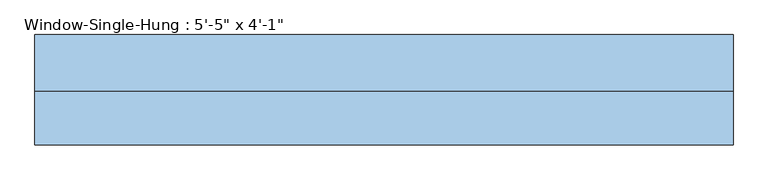
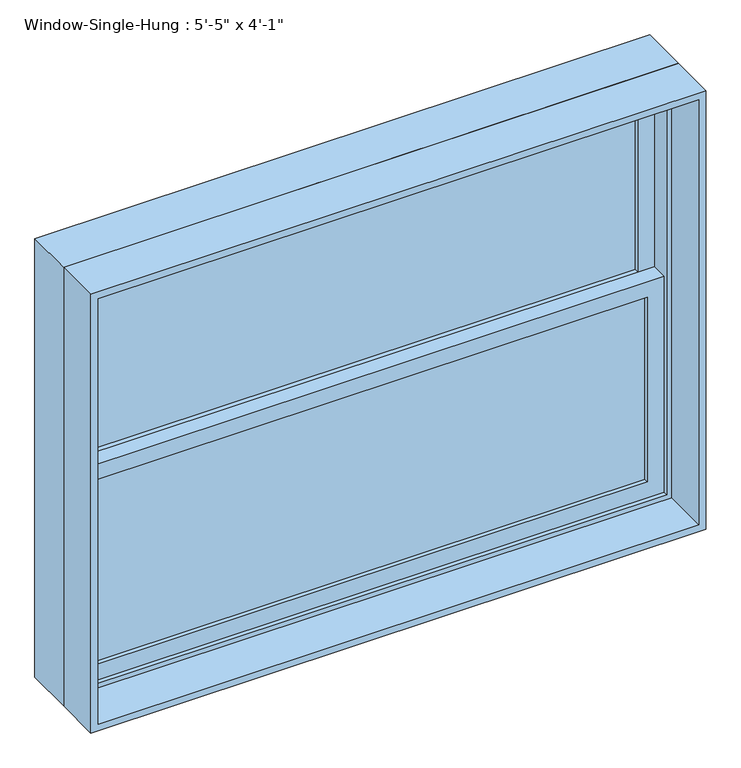
"""IFC4 building model written with IfcOpenShell, lengths in millimetres: window geometry."""

import ifcopenshell
import ifcopenshell.guid

model = None  # the IFC model being written
_history = None  # IfcOwnerHistory: only IFC2X3 demands one
_inside = {}  # id of a spatial element -> (the spatial element, [elements in it])
_under = {}  # id of a project, library or spatial element -> (it, [spatial elements below it])
_declared = {}  # id of a project -> (the project, [libraries it declares])
_typed = {}  # id of a type object -> (the type object, [elements of that type])
_made_of = {}  # id of a material, layer set ... -> (it, [elements and type objects made of it])


def new_model(schema):
    """Start an empty IFC model of exactly this schema.

    Asked for "IFC4X3", IfcOpenShell would pick the latest addendum, in which some entities
    have other attributes; the version numbers below select the first issue.
    IFC2X3 requires an IfcOwnerHistory on every rooted entity: one is made here for all.
    """
    global model, _history
    if schema == "IFC4X3":
        model = ifcopenshell.file(schema_version=(4, 3, 0, 0))
    else:
        model = ifcopenshell.file(schema=schema)
    _inside.clear()
    _under.clear()
    _declared.clear()
    _typed.clear()
    _made_of.clear()
    _history = None
    if model.schema == "IFC2X3":
        org = make("IfcOrganization", Name="unknown")
        user = make(
            "IfcPersonAndOrganization",
            ThePerson=make("IfcPerson", FamilyName="unknown"),
            TheOrganization=org,
        )
        app = make(
            "IfcApplication",
            ApplicationDeveloper=org,
            Version="unknown",
            ApplicationFullName="unknown",
            ApplicationIdentifier="unknown",
        )
        _history = make(
            "IfcOwnerHistory",
            OwningUser=user,
            OwningApplication=app,
            ChangeAction="ADDED",
            CreationDate=0,
        )
    return model


def make(cls, **values):
    """One entity of the class cls with the attributes given. An attribute that is None is left unset."""
    return model.create_entity(
        cls, **{name: value for name, value in values.items() if value is not None}
    )


def rooted(cls, **values):
    """An entity with a GlobalId (a new one), such as an element, a storey or a relation."""
    return make(cls, GlobalId=ifcopenshell.guid.new(), OwnerHistory=_history, **values)


def si_unit(unit_type, name, prefix=None):
    """IfcSIUnit, for example si_unit("LENGTHUNIT", "METRE", prefix="MILLI")."""
    return make("IfcSIUnit", UnitType=unit_type, Prefix=prefix, Name=name)


def assignment(units):
    """IfcUnitAssignment: the units of a project."""
    return None if units is None else make("IfcUnitAssignment", Units=units)


def point(xyz):
    """IfcCartesianPoint."""
    return None if xyz is None else make("IfcCartesianPoint", Coordinates=xyz)


def direction(xyz):
    """IfcDirection."""
    return None if xyz is None else make("IfcDirection", DirectionRatios=xyz)


def frame(location, z_axis=None, x_axis=None):
    """IfcAxis2Placement3D, a coordinate frame: its origin and axes. An axis left out is left unset."""
    return make(
        "IfcAxis2Placement3D",
        Location=point(location),
        Axis=direction(z_axis),
        RefDirection=direction(x_axis),
    )


def origin():
    """The frame at (0, 0, 0) with its axes left unset."""
    return frame((0.0, 0.0, 0.0))


def place(relative_to, where):
    """IfcLocalPlacement: puts the frame where relative to a parent placement (None: the world)."""
    return make(
        "IfcLocalPlacement", PlacementRelTo=relative_to, RelativePlacement=where
    )


def context(
    kind, dimensions, precision=None, world=None, true_north=None, identifier=None
):
    """IfcGeometricRepresentationContext, for example the 3D "Model" context."""
    return make(
        "IfcGeometricRepresentationContext",
        ContextIdentifier=identifier,
        ContextType=kind,
        CoordinateSpaceDimension=dimensions,
        Precision=precision,
        WorldCoordinateSystem=world,
        TrueNorth=true_north,
    )


def project(units=None, contexts=None):
    """IfcProject with its units and contexts."""
    return rooted(
        "IfcProject",
        Name="project",
        RepresentationContexts=contexts,
        UnitsInContext=assignment(units),
    )


def spatial(cls, under=None, at=None, **own):
    """A site, building, storey or space (cls), placed at a placement, below another one or the project."""
    s = rooted(cls, ObjectPlacement=at, **own)
    if under is not None:
        _under.setdefault(under.id(), (under, []))[1].append(s)
    return s


def polyline(points):
    """IfcPolyline through the points."""
    return make("IfcPolyline", Points=[point(p) for p in points])


def outline(outer, holes=None, kind="AREA"):
    """IfcArbitraryClosedProfileDef: a profile drawn as a closed curve; with holes, ...WithVoids."""
    if holes is None:
        return make("IfcArbitraryClosedProfileDef", ProfileType=kind, OuterCurve=outer)
    return make(
        "IfcArbitraryProfileDefWithVoids",
        ProfileType=kind,
        OuterCurve=outer,
        InnerCurves=holes,
    )


def extrude(swept, where, along, depth):
    """IfcExtrudedAreaSolid: the profile swept, set in the frame where, extruded along a direction by depth."""
    return make(
        "IfcExtrudedAreaSolid",
        SweptArea=swept,
        Position=where,
        ExtrudedDirection=direction(along),
        Depth=depth,
    )


def shape(context_of_items, identifier, shape_type, items):
    """IfcShapeRepresentation: the items that make up one representation, for example the "Body"."""
    return make(
        "IfcShapeRepresentation",
        ContextOfItems=context_of_items,
        RepresentationIdentifier=identifier,
        RepresentationType=shape_type,
        Items=items,
    )


def source(mapping_origin, context_of_items, identifier, shape_type, items):
    """IfcRepresentationMap: a shape defined once, which mapped items show again and again."""
    return make(
        "IfcRepresentationMap",
        MappingOrigin=mapping_origin,
        MappedRepresentation=shape(context_of_items, identifier, shape_type, items),
    )


def transform(
    local_origin,
    x_axis=None,
    y_axis=None,
    z_axis=None,
    scale=None,
    scale2=None,
    scale3=None,
    uniform=True,
):
    """IfcCartesianTransformationOperator3D, or its non-uniform kind. x_axis, y_axis, z_axis: its Axis1, 2, 3."""
    if uniform:
        return make(
            "IfcCartesianTransformationOperator3D",
            Axis1=direction(x_axis),
            Axis2=direction(y_axis),
            LocalOrigin=point(local_origin),
            Scale=scale,
            Axis3=direction(z_axis),
        )
    return make(
        "IfcCartesianTransformationOperator3DnonUniform",
        Axis1=direction(x_axis),
        Axis2=direction(y_axis),
        LocalOrigin=point(local_origin),
        Scale=scale,
        Axis3=direction(z_axis),
        Scale2=scale2,
        Scale3=scale3,
    )


def mapped(mapping_source, mapping_target):
    """IfcMappedItem: shows the shape of a source again, moved by a transform."""
    return make(
        "IfcMappedItem", MappingSource=mapping_source, MappingTarget=mapping_target
    )


def made_of(thing, what):
    """Note that an element or type object is made of a material, layer set ...; save() writes the relation."""
    if what is not None:
        _made_of.setdefault(what.id(), (what, []))[1].append(thing)
    return thing


def element(
    cls,
    number,
    at=None,
    inside=None,
    cuts=None,
    type_object=None,
    material=None,
    context=None,
    identifier="Body",
    shape_type=None,
    held_by="IfcProductDefinitionShape",
    body=None,
    shapes=None,
    **own,
):
    """One element of the class cls, such as IfcWall. Its Tag is "e" and its number.

    at: its placement. inside: the storey or other place that contains it. cuts: it is an
    opening in that element (IfcRelVoidsElement). A single representation is given by context,
    identifier, shape_type and body (its items); several are given by shapes. held_by: the class
    of the entity that holds the representations. save() writes the other relations.
    """
    e = rooted(cls, Tag="e%d" % number, ObjectPlacement=at, **own)
    if body is not None:
        shapes = [shape(context, identifier, shape_type, body)]
    if shapes is not None:
        e.Representation = make(held_by, Representations=shapes)
    if inside is not None:
        _inside.setdefault(inside.id(), (inside, []))[1].append(e)
    if cuts is not None:
        rooted(
            "IfcRelVoidsElement", RelatingBuildingElement=cuts, RelatedOpeningElement=e
        )
    if type_object is not None:
        _typed.setdefault(type_object.id(), (type_object, []))[1].append(e)
    return made_of(e, material)


def aggregate(whole, parts):
    """IfcRelAggregates: a whole, such as a stair, and the parts it consists of."""
    return rooted("IfcRelAggregates", RelatingObject=whole, RelatedObjects=parts)


def save(model, path):
    """Write the relations noted so far, then the file.

    IfcRelAggregates (storeys below a building ...), IfcRelContainedInSpatialStructure (elements
    in a storey), IfcRelDefinesByType, IfcRelAssociatesMaterial and IfcRelDeclares: one each for
    every whole, place, type object, material and project.
    """
    for whole, parts in _under.values():
        aggregate(whole, parts)
    for where, things in _inside.values():
        rooted(
            "IfcRelContainedInSpatialStructure",
            RelatedElements=things,
            RelatingStructure=where,
        )
    for kind, things in _typed.values():
        rooted("IfcRelDefinesByType", RelatedObjects=things, RelatingType=kind)
    for what, things in _made_of.values():
        rooted("IfcRelAssociatesMaterial", RelatedObjects=things, RelatingMaterial=what)
    for by, libraries in _declared.values():
        rooted("IfcRelDeclares", RelatingContext=by, RelatedDefinitions=libraries)
    model.write(path)


def window_21bbe75a(model_context):
    return source(origin(), model_context, "Body", "SweptSolid", [
        extrude(outline(polyline([(749.3, 50.8), (749.3, 44.45), (-749.3, 44.45), (-749.3, 50.8), (749.3, 50.8)])), frame((0.0, 0.0, 990.6), z_axis=(0.0, 0.0, 1.0), x_axis=(1.0, 0.0, 0.0)), (0.0, 0.0, 1.0), 523.875),
        extrude(outline(polyline([(-749.3, 38.1), (749.3, 38.1), (749.3, 31.75), (-749.3, 31.75), (-749.3, 38.1)])), frame((0.0, 0.0, 990.6), z_axis=(0.0, 0.0, 1.0), x_axis=(1.0, 0.0, 0.0)), (0.0, 0.0, 1.0), 523.875),
        extrude(outline(polyline([(749.3, 95.25), (749.3, 88.9), (-749.3, 88.9), (-749.3, 95.25), (749.3, 95.25)])), frame((0.0, 0.0, 1558.925), z_axis=(0.0, 0.0, 1.0), x_axis=(1.0, 0.0, 0.0)), (0.0, 0.0, 1.0), 523.875),
        extrude(outline(polyline([(-749.3, 82.55), (749.3, 82.55), (749.3, 76.2), (-749.3, 76.2), (-749.3, 82.55)])), frame((0.0, 0.0, 1558.925), z_axis=(0.0, 0.0, 1.0), x_axis=(1.0, 0.0, 0.0)), (0.0, 0.0, 1.0), 523.875),
        extrude(outline(polyline([(1558.925, -793.75), (946.15, -793.75), (946.15, 793.75), (1558.925, 793.75), (1558.925, -793.75)]), holes=[polyline([(1514.475, 749.3), (990.6, 749.3), (990.6, -749.3), (1514.475, -749.3), (1514.475, 749.3)])]), frame((0.0, 19.05, 0.0), z_axis=(0.0, 1.0, 0.0), x_axis=(0.0, 0.0, 1.0)), (0.0, 0.0, 1.0), 44.45),
        extrude(outline(polyline([(2127.25, -793.75), (1514.475, -793.75), (1514.475, 793.75), (2127.25, 793.75), (2127.25, -793.75)]), holes=[polyline([(2082.8, 749.3), (1558.925, 749.3), (1558.925, -749.3), (2082.8, -749.3), (2082.8, 749.3)])]), frame((0.0, 63.5, 0.0), z_axis=(0.0, 1.0, 0.0), x_axis=(0.0, 0.0, 1.0)), (0.0, 0.0, 1.0), 44.45),
        extrude(outline(polyline([(2159.0, -825.5), (914.4, -825.5), (914.4, 825.5), (2159.0, 825.5), (2159.0, -825.5)]), holes=[polyline([(2127.25, 793.75), (946.15, 793.75), (946.15, -793.75), (2127.25, -793.75), (2127.25, 793.75)])]), frame((0.0, 6.35, 0.0), z_axis=(0.0, 1.0, 0.0), x_axis=(0.0, 0.0, 1.0)), (0.0, 0.0, 1.0), 133.35),
        extrude(outline(polyline([(2159.0, 825.5), (2159.0, -825.5), (914.4, -825.5), (914.4, 825.5), (2159.0, 825.5)]), holes=[polyline([(2139.95, 806.45), (933.45, 806.45), (933.45, -806.45), (2139.95, -806.45), (2139.95, 806.45)])]), frame((0.0, -120.65, 0.0), z_axis=(0.0, 1.0, 0.0), x_axis=(0.0, 0.0, 1.0)), (0.0, 0.0, 1.0), 127.0),
    ])


if __name__ == "__main__":
    model = new_model("IFC4")
    model_context = context("Model", 3, world=origin())
    ifc_project = project(units=[si_unit("LENGTHUNIT", "METRE", prefix="MILLI")], contexts=[model_context])
    site = spatial("IfcSite", under=ifc_project)
    building = spatial("IfcBuilding", under=site)
    placement = place(None, origin())
    window_shape = window_21bbe75a(model_context)
    element("IfcWindow", 1, ObjectType="Window-Single-Hung : 5'-5\" x 4'-1\"", at=placement, inside=building, context=model_context, shape_type="MappedRepresentation", body=[
        mapped(window_shape, transform((0.0, 0.0, 0.0), x_axis=(1.0, 0.0, 0.0), y_axis=(0.0, 1.0, 0.0), z_axis=(0.0, 0.0, 1.0))),
    ])
    save(model, "model.ifc")

# Revit data of these elements
# Type "Window-Single-Hung : 5'-5\" x 4'-1\""
#   Type Mark = "27"
#   Fire Rating = "0.5h"
#   Construction Type Id = "DG-DR"
#   Assembly Code = "B2020100"
#   Analytic Construction = "Double glazing - domestic"
#   Wall Thickness [instance default] = 0' - 6"
#   Window Inset [instance default] = 0' - 0"
#   Visual Light Transmittance = 0.81
#   Thermal Resistance (R) = 0.319569 (m²·K)/W
#   Solar Heat Gain Coefficient = 0.76
#   Muntin Width = 4' - 11"
#   Muntin Height = 1' - 8 5/8"
#   Interior Wall Closure [instance default] = 0' - 1 1/2"
#   Rough Width = 5' - 5 1/2"
#   Rough Height = 4' - 1 1/2"
#   Frame Extension [instance default] = 0' - 1 1/4"
#   Exterior Wall Closure [instance default] = 0' - 0 1/2"
#   Extension Jamb [instance default] = 0' - 1 1/2"
#   Heat Transfer Coefficient (U) = 3.12929 W/(m²·K)
#   Height = 4' - 1"
#   Width = 5' - 5"
#   Top Muntin Visibility = yes
#   Indicator Visibility [instance default] = yes
#   Extension Jamb Visibility [instance default] = yes
#   Interior Trim Visibility [instance default] = yes
#   Exterior Trim Visibility [instance default] = yes
#   Bottom Muntin Visibility = yes
#   Muntin Pattern = Muntin Pattern_2x2 : Muntin Pattern_2x2
#   Interior Trim Material = Wood - Stained
#   Interior Trim = Trim-Window-Interior-Flat : Picture Frame
#   Exterior Trim Material = Clad - White
#   Exterior Trim = Trim-Window-Exterior-Flat : with Sill
#   Glass Panel Material = Glass
#   Exterior Frame Material = Clad - White
#   Interior Frame Material = Wood - Stained
#   Wall Closure = (empty or 0)
# Element 1 (IfcWindow, "Window-Single-Hung : 5'-5\" x 4'-1\"")
#   Wall Thickness = 0' - 9 1/2"
#   Extension Jamb = 0' - 5"
#   Materials on its faces: "Wood - Stained", "Glass", "Clad - White"
# Materials
#   "Wood - Stained": class "Wood", colour RGB 224 178 126, transparency 0, Cost = 0
#   "Clad - White": class "Wood", colour RGB 242 242 238, transparency 0, Cost = 0
#   "Glass": class "Glass", colour RGB 218 227 224, transparency 0.85, Description = "Soda Lime Glass", Cost = 0
